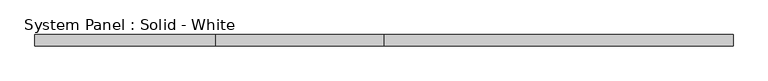
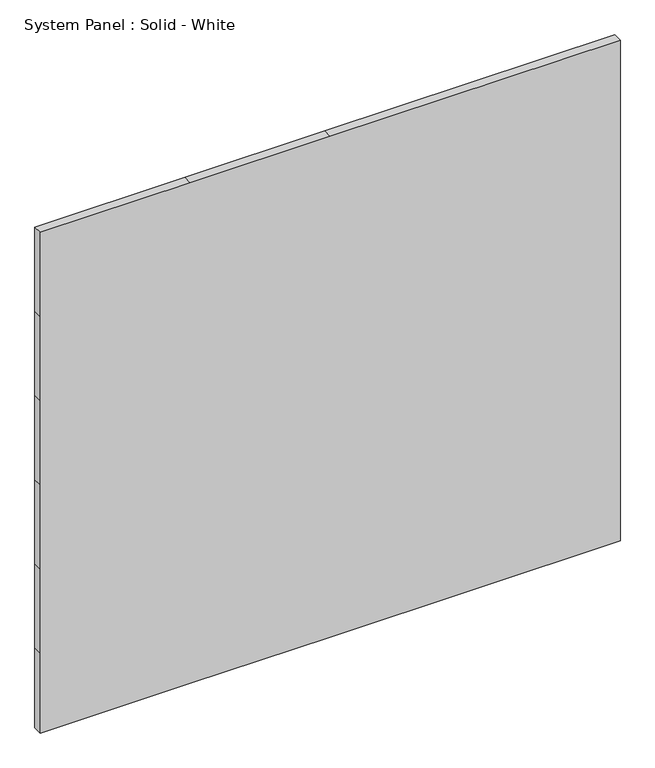
"""IFC4 building model written with IfcOpenShell, lengths in millimetres: plate geometry, System Panel : Solid - White."""

from ifc_helpers import new_model, si_unit, frame, origin, place, context, project, spatial, polyline, outline, extrude, source, transform, mapped, element, save


def system_panel_solid_white_9196c263(model_context):
    return source(origin(), model_context, "Body", "SweptSolid", [
        extrude(outline(polyline([(0.0, -1987.55), (0.0, -958.85), (0.0, 0.0), (0.0, 1987.55), (577.85, 1987.55), (1187.45, 1987.55), (1797.05, 1987.55), (2406.65, 1987.55), (3016.25, 1987.55), (3625.85, 1987.55), (3625.85, 0.0), (3625.85, -958.85), (3625.85, -1987.55), (3016.25, -1987.55), (2406.65, -1987.55), (1797.05, -1987.55), (1187.45, -1987.55), (577.85, -1987.55), (0.0, -1987.55)])), frame((0.0, -19.05, 0.0), z_axis=(0.0, 1.0, 0.0), x_axis=(0.0, 0.0, 1.0)), (0.0, 0.0, 1.0), 63.5),
    ])


if __name__ == "__main__":
    model = new_model("IFC4")
    model_context = context("Model", 3, world=origin())
    ifc_project = project(units=[si_unit("LENGTHUNIT", "METRE", prefix="MILLI")], contexts=[model_context])
    site = spatial("IfcSite", under=ifc_project)
    building = spatial("IfcBuilding", under=site)
    placement = place(None, origin())
    system_panel_solid_white_shape = system_panel_solid_white_9196c263(model_context)
    element("IfcPlate", 1, ObjectType="System Panel : Solid - White", at=placement, inside=building, context=model_context, shape_type="MappedRepresentation", body=[
        mapped(system_panel_solid_white_shape, transform((0.0, 0.0, 0.0), x_axis=(1.0, 0.0, 0.0), y_axis=(0.0, 1.0, 0.0), z_axis=(0.0, 0.0, 1.0))),
    ])
    save(model, "model.ifc")

# Revit data of these elements
# Element 1 (IfcPlate, "System Panel : Solid - White")
#   Materials on its faces: "White Panel"
# Materials
#   "White Panel": class "Unassigned", colour RGB 255 255 255, transparency 0
